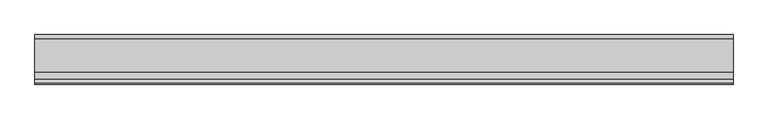
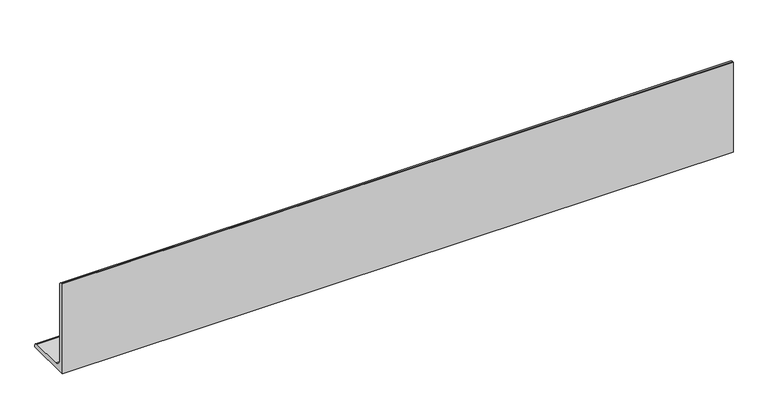
"""IFC4 building model written with IfcOpenShell, lengths in millimetres: beam geometry, NLRS_28_SF_LIB_stalen ligger hoekprofiel ongelijkzijdig-AV-MMBS-SRP_gen_rsf : stalen ligger ongelijzijdig hoekprofiel LUEQ_gen__200x100x10."""

from ifc_helpers import new_model, si_unit, point, frame, frame_2d, origin, place, context, project, spatial, polyline, circle_curve, trimmed, segment, composite_curve, outline, extrude, source, transform, mapped, element, save


def beam_7c957b24(model_context):
    return source(origin(), model_context, "Body", "SweptSolid", [
        extrude(outline(composite_curve([segment(polyline([(-20.13, -69.3), (-20.13, 130.7), (-17.63, 130.7)]), True, "CONTINUOUS"), segment(trimmed(circle_curve(frame_2d((-17.63, 123.2)), 7.5), [point((-17.63, 130.7))], [point((-10.13, 123.2))], False, "CARTESIAN"), True, "CONTINUOUS"), segment(polyline([(-10.13, 123.2), (-10.13, -44.3)]), True, "CONTINUOUS"), segment(trimmed(circle_curve(frame_2d((4.87, -44.3)), 15.0), [point((-10.13, -44.3))], [point((4.87, -59.3))], True, "CARTESIAN"), True, "CONTINUOUS"), segment(polyline([(4.87, -59.3), (72.37, -59.3)]), True, "CONTINUOUS"), segment(trimmed(circle_curve(frame_2d((72.37, -66.8)), 7.5), [point((72.37, -59.3))], [point((79.87, -66.8))], False, "CARTESIAN"), True, "CONTINUOUS"), segment(polyline([(79.87, -66.8), (79.87, -69.3), (-20.13, -69.3)]), True, "CONTINUOUS")], self_intersect=False)), frame((-710.0, 0.0, 0.0), z_axis=(1.0, 0.0, 0.0), x_axis=(0.0, 1.0, 0.0)), (0.0, 0.0, 1.0), 1407.2999994),
    ])


if __name__ == "__main__":
    model = new_model("IFC4")
    model_context = context("Model", 3, world=origin())
    ifc_project = project(units=[si_unit("LENGTHUNIT", "METRE", prefix="MILLI")], contexts=[model_context])
    site = spatial("IfcSite", under=ifc_project)
    building = spatial("IfcBuilding", under=site)
    placement = place(None, origin())
    beam_shape = beam_7c957b24(model_context)
    element("IfcBeam", 1, ObjectType="NLRS_28_SF_LIB_stalen ligger hoekprofiel ongelijkzijdig-AV-MMBS-SRP_gen_rsf : stalen ligger ongelijzijdig hoekprofiel LUEQ_gen__200x100x10", at=placement, inside=building, context=model_context, shape_type="MappedRepresentation", body=[
        mapped(beam_shape, transform((0.0, 0.0, 0.0), x_axis=(1.0, 0.0, 0.0), y_axis=(0.0, 1.0, 0.0), z_axis=(0.0, 0.0, 1.0))),
    ])
    save(model, "model.ifc")

# Revit data of these elements
# Type "NLRS_28_SF_LIB_stalen ligger hoekprofiel ongelijkzijdig-AV-MMBS-SRP_gen_rsf : stalen ligger ongelijzijdig hoekprofiel LUEQ_gen__200x100x10"
#   Type IfcGUID = "0dxhH9VHH5jh7XQ0uLfXuR"
#   IfcExportAs = "IfcBeamType"
#   Type Comments = "L200x100x10"
#   Model = " "
#   Manufacturer = " "
#   Fire Rating = " "
#   Description = "stalen ligger L200x100x10"
#   Assembly Code = "28.11"
#   vz = 130.7 mm
#   vy = 79.87 mm
#   tw = 10 mm
#   tf = 10 mm
#   ri = 7.5 mm
#   ra = 15 mm
#   d = 200 mm
#   bf = 100 mm
#   NLRS_C_lengte [instance default] = 1524 mm
#   Length [instance default] = 1524 mm
#   Structural Material = NLRS_h2_staal_gen_rsf
#   Keynote = ""
# Element 1 (IfcBeam, "NLRS_28_SF_LIB_stalen ligger hoekprofiel ongelijkzijdig-AV-MMBS-SRP_gen_rsf : stalen ligger ongelijzijdig hoekprofiel LUEQ_gen__200x100x10")
#   NLRS_C_lengte = 1420 mm
#   Materials on its faces: "NLRS_h2_staal_gen_rsf"
# Materials
#   "NLRS_h2_staal_gen_rsf": class "H - Metaal", colour RGB 189 187 185, transparency 0, Keynote = "h2", Manufacturer = "Revit Standards Foundation", URL = "www.revitstandards.org", Description = "staal", Cost = 0
